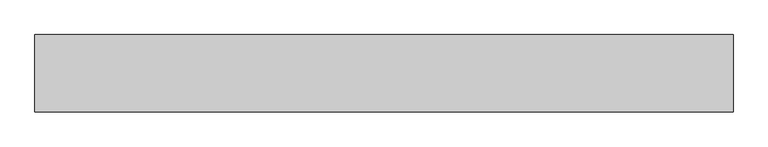
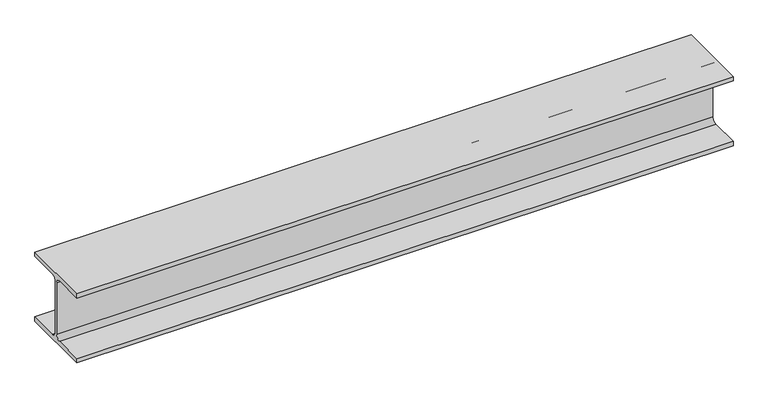
"""IFC4 building model written with IfcOpenShell, lengths in millimetres: beam geometry, 0912_Steel Framing_H-KSD3502 : H_SB_ASB_H-200x200x8x12."""

from ifc_helpers import new_model, si_unit, point, frame, frame_2d, origin, place, context, project, spatial, polyline, circle_curve, trimmed, segment, composite_curve, outline, extrude, source, transform, mapped, element, save


def beam_275389fa(model_context):
    return source(origin(), model_context, "Body", "SweptSolid", [
        extrude(outline(composite_curve([segment(polyline([(100.0, -88.0), (100.0, -100.0), (-100.0, -100.0), (-100.0, -88.0), (-17.0, -88.0)]), True, "CONTINUOUS"), segment(trimmed(circle_curve(frame_2d((-17.0, -75.0)), 13.0), [point((-17.0, -88.0))], [point((-4.0, -75.0))], True, "CARTESIAN"), True, "CONTINUOUS"), segment(polyline([(-4.0, -75.0), (-4.0, 75.0)]), True, "CONTINUOUS"), segment(trimmed(circle_curve(frame_2d((-17.0, 75.0)), 13.0), [point((-4.0, 75.0))], [point((-17.0, 88.0))], True, "CARTESIAN"), True, "CONTINUOUS"), segment(polyline([(-17.0, 88.0), (-100.0, 88.0), (-100.0, 100.0), (100.0, 100.0), (100.0, 88.0), (17.0, 88.0)]), True, "CONTINUOUS"), segment(trimmed(circle_curve(frame_2d((17.0, 75.0)), 13.0), [point((17.0, 88.0))], [point((4.0, 75.0))], True, "CARTESIAN"), True, "CONTINUOUS"), segment(polyline([(4.0, 75.0), (4.0, -75.0)]), True, "CONTINUOUS"), segment(trimmed(circle_curve(frame_2d((17.0, -75.0)), 13.0), [point((4.0, -75.0))], [point((17.0, -88.0))], True, "CARTESIAN"), True, "CONTINUOUS"), segment(polyline([(17.0, -88.0), (100.0, -88.0)]), True, "CONTINUOUS")], self_intersect=False)), frame((-827.130962, 0.0, 0.0), z_axis=(1.0, 0.0, 0.0), x_axis=(0.0, 1.0, 0.0)), (0.0, 0.0, 1.0), 1801.7481877),
    ])


if __name__ == "__main__":
    model = new_model("IFC4")
    model_context = context("Model", 3, world=origin())
    ifc_project = project(units=[si_unit("LENGTHUNIT", "METRE", prefix="MILLI")], contexts=[model_context])
    site = spatial("IfcSite", under=ifc_project)
    building = spatial("IfcBuilding", under=site)
    placement = place(None, origin())
    beam_shape = beam_275389fa(model_context)
    element("IfcBeam", 1, ObjectType="0912_Steel Framing_H-KSD3502 : H_SB_ASB_H-200x200x8x12", at=placement, inside=building, context=model_context, shape_type="MappedRepresentation", body=[
        mapped(beam_shape, transform((0.0, 0.0, 0.0), x_axis=(1.0, 0.0, 0.0), y_axis=(0.0, 1.0, 0.0), z_axis=(0.0, 0.0, 1.0))),
    ])
    save(model, "model.ifc")

# Revit data of these elements
# Type "0912_Steel Framing_H-KSD3502 : H_SB_ASB_H-200x200x8x12"
#   H_WM Code_1 = "S01AA002-00001 | Main Steel Structure Fabrication Work | Shelter/Building | Medium Steel - Standard (90KG/M>Weight≥30KG/M) | Material: (   )"
#   H_WM Code_2 = "S03AA028-00001 | Main Steel Structure Erection Work | Shelter/Building | Medium Steel (90KG/M>Weight≥30KG/M) | Material: (   )"
#   H_WM Code_3 = "S01AA010-00001 | Main Steel Structure Fabrication Work | Shelter/Building | Steel Painting/Coating | for Non-Fireproofed Steel Surface, Surface Preparation, Primer, Second & Final Coat | Material: (   )"
#   H_Q'ty Cal Type Tag = "SB-Q2"
#   Width = 20.0 cm
#   Web Thickness = 0.8 cm
#   Web Fillet = 1.3 cm
#   Warping Constant = 141000.0 cm⁶
#   W = 0
#   Torsional Moment of Inertia = 26.2485 cm⁴
#   Section Area = 63.53 cm²
#   Plastic Modulus weak axis = 244.0 cm³
#   Plastic Modulus strong axis = 525.0 cm³
#   Perimeter = 1.16 m²/m
#   Nominal Weight = 49.90 kgf/m
#   Moment of Inertia weak axis = 1600.00 cm⁴
#   Moment of Inertia strong axis = 4720.00 cm⁴
#   Height = 20.0 cm
#   Flange Thickness = 1.2 cm
#   Elastic Modulus weak axis = 160.0 cm³
#   Elastic Modulus strong axis = 472.0 cm³
#   Centroid Vertical = 10.0 cm
#   Centroid Horizontal = 10.0 cm
#   Ix = 47200000
#   Length [instance default] = 1.5240 m
#   Zx = 525000
#   b = 0.2000 m
#   h = 0.2000 m
#   r = 0.0130 m
#   s = 0.0080 m
#   t = 0.0120 m
#   A = 0.006353 m²
#   Structural Material [instance default] = Steel, 45-345
#   Assembly Code = ""
# Element 1 (IfcBeam, "0912_Steel Framing_H-KSD3502 : H_SB_ASB_H-200x200x8x12")
#   Structural Material = none
# Materials
#   "Steel, 45-345": class "Metal", colour RGB 189 187 185, transparency 0, Description = "Steel 345 MPa", Cost = 0
